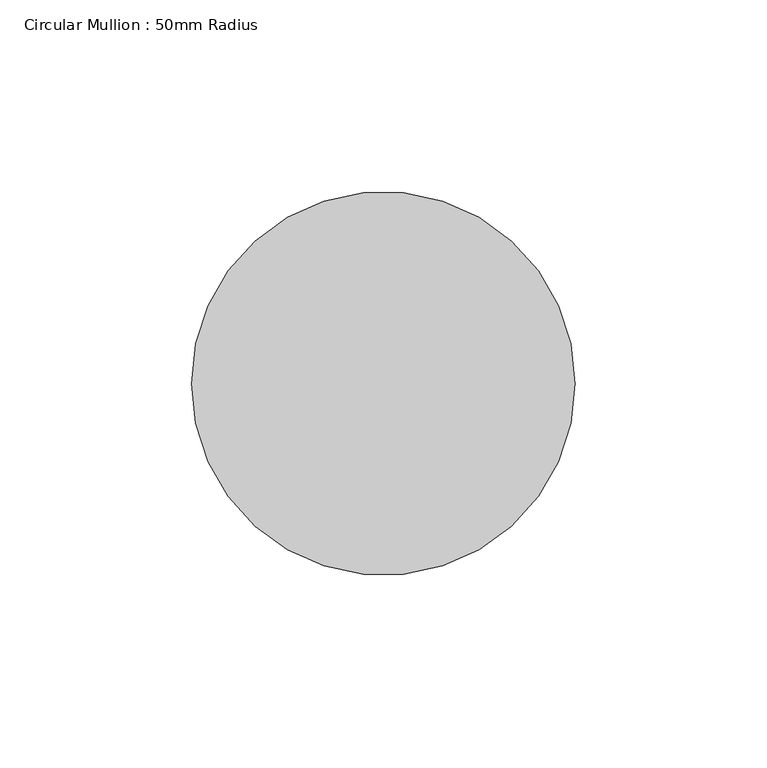
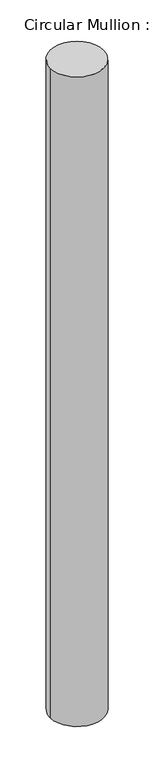
"""IFC4 building model written with IfcOpenShell, lengths in millimetres: member geometry, Circular Mullion : 50mm Radius."""

from ifc_helpers import new_model, si_unit, point, frame, origin, origin_2d, place, context, project, spatial, circle_curve, trimmed, segment, composite_curve, outline, extrude, source, transform, mapped, element, save


def circular_mullion_50mm_radius_ec13de1c(model_context):
    return source(origin(), model_context, "Body", "SweptSolid", [
        extrude(outline(composite_curve([segment(trimmed(circle_curve(origin_2d(), 50.0), [point((50.0, 0.0))], [point((-50.0, 0.0))], False, "CARTESIAN"), True, "CONTINUOUS"), segment(trimmed(circle_curve(origin_2d(), 50.0), [point((-50.0, 0.0))], [point((50.0, 0.0))], False, "CARTESIAN"), True, "CONTINUOUS")], self_intersect=False)), frame((0.0, 0.0, -1281.1470511), z_axis=(0.0, 0.0, 1.0), x_axis=(1.0, 0.0, 0.0)), (0.0, 0.0, 1.0), 1281.1470511),
    ])


if __name__ == "__main__":
    model = new_model("IFC4")
    model_context = context("Model", 3, world=origin())
    ifc_project = project(units=[si_unit("LENGTHUNIT", "METRE", prefix="MILLI")], contexts=[model_context])
    site = spatial("IfcSite", under=ifc_project)
    building = spatial("IfcBuilding", under=site)
    placement = place(None, origin())
    circular_mullion_50mm_radius_shape = circular_mullion_50mm_radius_ec13de1c(model_context)
    element("IfcMember", 1, ObjectType="Circular Mullion : 50mm Radius", at=placement, inside=building, context=model_context, shape_type="MappedRepresentation", body=[
        mapped(circular_mullion_50mm_radius_shape, transform((0.0, 0.0, 0.0), x_axis=(1.0, 0.0, 0.0), y_axis=(0.0, 1.0, 0.0), z_axis=(0.0, 0.0, 1.0))),
    ])
    save(model, "model.ifc")

# Revit data of these elements
# Type "Circular Mullion : 50mm Radius"
#   built-in parameter 1007350 = 0.164042 (stored number, unit not read)
# Element 1 (IfcMember, "Circular Mullion : 50mm Radius")
#   Materials on its faces: "Aluminium"
# Materials
#   "Aluminium": class "Metal", colour RGB 247 247 247, transparency 0, Description = "Aluminium 6061", Cost = 0
